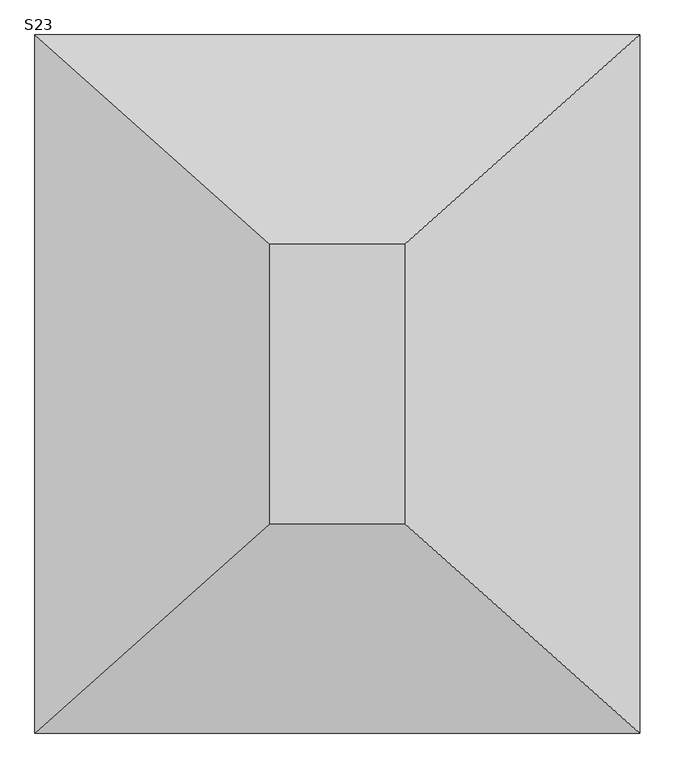
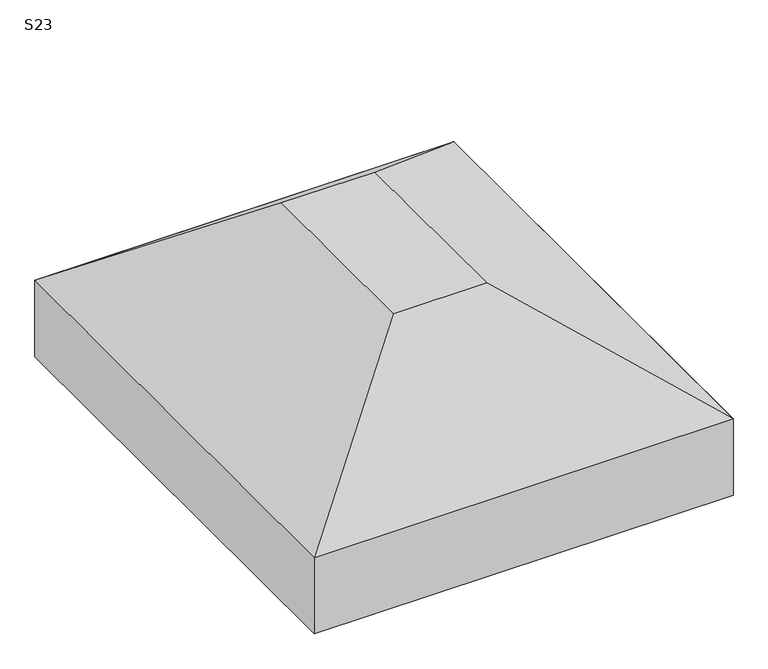
"""IFC4 building model written with IfcOpenShell, lengths in millimetres: fastener geometry, TQS - Sapata : S23."""

import ifcopenshell
import ifcopenshell.guid

model = None  # the IFC model being written
_history = None  # IfcOwnerHistory: only IFC2X3 demands one
_inside = {}  # id of a spatial element -> (the spatial element, [elements in it])
_under = {}  # id of a project, library or spatial element -> (it, [spatial elements below it])
_declared = {}  # id of a project -> (the project, [libraries it declares])
_typed = {}  # id of a type object -> (the type object, [elements of that type])
_made_of = {}  # id of a material, layer set ... -> (it, [elements and type objects made of it])


def new_model(schema):
    """Start an empty IFC model of exactly this schema.

    Asked for "IFC4X3", IfcOpenShell would pick the latest addendum, in which some entities
    have other attributes; the version numbers below select the first issue.
    IFC2X3 requires an IfcOwnerHistory on every rooted entity: one is made here for all.
    """
    global model, _history
    if schema == "IFC4X3":
        model = ifcopenshell.file(schema_version=(4, 3, 0, 0))
    else:
        model = ifcopenshell.file(schema=schema)
    _inside.clear()
    _under.clear()
    _declared.clear()
    _typed.clear()
    _made_of.clear()
    _history = None
    if model.schema == "IFC2X3":
        org = make("IfcOrganization", Name="unknown")
        user = make(
            "IfcPersonAndOrganization",
            ThePerson=make("IfcPerson", FamilyName="unknown"),
            TheOrganization=org,
        )
        app = make(
            "IfcApplication",
            ApplicationDeveloper=org,
            Version="unknown",
            ApplicationFullName="unknown",
            ApplicationIdentifier="unknown",
        )
        _history = make(
            "IfcOwnerHistory",
            OwningUser=user,
            OwningApplication=app,
            ChangeAction="ADDED",
            CreationDate=0,
        )
    return model


def make(cls, **values):
    """One entity of the class cls with the attributes given. An attribute that is None is left unset."""
    return model.create_entity(
        cls, **{name: value for name, value in values.items() if value is not None}
    )


def rooted(cls, **values):
    """An entity with a GlobalId (a new one), such as an element, a storey or a relation."""
    return make(cls, GlobalId=ifcopenshell.guid.new(), OwnerHistory=_history, **values)


def si_unit(unit_type, name, prefix=None):
    """IfcSIUnit, for example si_unit("LENGTHUNIT", "METRE", prefix="MILLI")."""
    return make("IfcSIUnit", UnitType=unit_type, Prefix=prefix, Name=name)


def assignment(units):
    """IfcUnitAssignment: the units of a project."""
    return None if units is None else make("IfcUnitAssignment", Units=units)


def point(xyz):
    """IfcCartesianPoint."""
    return None if xyz is None else make("IfcCartesianPoint", Coordinates=xyz)


def direction(xyz):
    """IfcDirection."""
    return None if xyz is None else make("IfcDirection", DirectionRatios=xyz)


def frame(location, z_axis=None, x_axis=None):
    """IfcAxis2Placement3D, a coordinate frame: its origin and axes. An axis left out is left unset."""
    return make(
        "IfcAxis2Placement3D",
        Location=point(location),
        Axis=direction(z_axis),
        RefDirection=direction(x_axis),
    )


def origin():
    """The frame at (0, 0, 0) with its axes left unset."""
    return frame((0.0, 0.0, 0.0))


def place(relative_to, where):
    """IfcLocalPlacement: puts the frame where relative to a parent placement (None: the world)."""
    return make(
        "IfcLocalPlacement", PlacementRelTo=relative_to, RelativePlacement=where
    )


def context(
    kind, dimensions, precision=None, world=None, true_north=None, identifier=None
):
    """IfcGeometricRepresentationContext, for example the 3D "Model" context."""
    return make(
        "IfcGeometricRepresentationContext",
        ContextIdentifier=identifier,
        ContextType=kind,
        CoordinateSpaceDimension=dimensions,
        Precision=precision,
        WorldCoordinateSystem=world,
        TrueNorth=true_north,
    )


def project(units=None, contexts=None):
    """IfcProject with its units and contexts."""
    return rooted(
        "IfcProject",
        Name="project",
        RepresentationContexts=contexts,
        UnitsInContext=assignment(units),
    )


def spatial(cls, under=None, at=None, **own):
    """A site, building, storey or space (cls), placed at a placement, below another one or the project."""
    s = rooted(cls, ObjectPlacement=at, **own)
    if under is not None:
        _under.setdefault(under.id(), (under, []))[1].append(s)
    return s


def polyline(points):
    """IfcPolyline through the points."""
    return make("IfcPolyline", Points=[point(p) for p in points])


def outline(outer, holes=None, kind="AREA"):
    """IfcArbitraryClosedProfileDef: a profile drawn as a closed curve; with holes, ...WithVoids."""
    if holes is None:
        return make("IfcArbitraryClosedProfileDef", ProfileType=kind, OuterCurve=outer)
    return make(
        "IfcArbitraryProfileDefWithVoids",
        ProfileType=kind,
        OuterCurve=outer,
        InnerCurves=holes,
    )


def extrude(swept, where, along, depth):
    """IfcExtrudedAreaSolid: the profile swept, set in the frame where, extruded along a direction by depth."""
    return make(
        "IfcExtrudedAreaSolid",
        SweptArea=swept,
        Position=where,
        ExtrudedDirection=direction(along),
        Depth=depth,
    )


def faces_of(points, faces, orient=None, outer=None):
    """IfcFace entities. A face is a list of loops; a loop is a list of indices into points, from 0.

    orient and outer hold one flag for each loop. By default every Orientation is true, the
    first loop of a face is its IfcFaceOuterBound and the others are IfcFaceBound.
    """
    made = []
    for i, loops in enumerate(faces):
        bounds = []
        for j, loop in enumerate(loops):
            is_outer = j == 0 if outer is None else outer[i][j]
            bounds.append(
                make(
                    "IfcFaceOuterBound" if is_outer else "IfcFaceBound",
                    Bound=make("IfcPolyLoop", Polygon=[points[k] for k in loop]),
                    Orientation=True if orient is None else orient[i][j],
                )
            )
        made.append(make("IfcFace", Bounds=bounds))
    return made


def faceted_brep(points, faces, orient=None, outer=None, voids=None):
    """IfcFacetedBrep: a solid bounded by flat faces; with voids (closed shells), ...WithVoids."""
    shared = [point(p) for p in points]
    hull = make("IfcClosedShell", CfsFaces=faces_of(shared, faces, orient, outer))
    if voids is None:
        return make("IfcFacetedBrep", Outer=hull)
    return make(
        "IfcFacetedBrepWithVoids",
        Outer=hull,
        Voids=[
            make(cls, CfsFaces=faces_of(shared, fs, o, b)) for cls, fs, o, b in voids
        ],
    )


def shape(context_of_items, identifier, shape_type, items):
    """IfcShapeRepresentation: the items that make up one representation, for example the "Body"."""
    return make(
        "IfcShapeRepresentation",
        ContextOfItems=context_of_items,
        RepresentationIdentifier=identifier,
        RepresentationType=shape_type,
        Items=items,
    )


def source(mapping_origin, context_of_items, identifier, shape_type, items):
    """IfcRepresentationMap: a shape defined once, which mapped items show again and again."""
    return make(
        "IfcRepresentationMap",
        MappingOrigin=mapping_origin,
        MappedRepresentation=shape(context_of_items, identifier, shape_type, items),
    )


def transform(
    local_origin,
    x_axis=None,
    y_axis=None,
    z_axis=None,
    scale=None,
    scale2=None,
    scale3=None,
    uniform=True,
):
    """IfcCartesianTransformationOperator3D, or its non-uniform kind. x_axis, y_axis, z_axis: its Axis1, 2, 3."""
    if uniform:
        return make(
            "IfcCartesianTransformationOperator3D",
            Axis1=direction(x_axis),
            Axis2=direction(y_axis),
            LocalOrigin=point(local_origin),
            Scale=scale,
            Axis3=direction(z_axis),
        )
    return make(
        "IfcCartesianTransformationOperator3DnonUniform",
        Axis1=direction(x_axis),
        Axis2=direction(y_axis),
        LocalOrigin=point(local_origin),
        Scale=scale,
        Axis3=direction(z_axis),
        Scale2=scale2,
        Scale3=scale3,
    )


def mapped(mapping_source, mapping_target):
    """IfcMappedItem: shows the shape of a source again, moved by a transform."""
    return make(
        "IfcMappedItem", MappingSource=mapping_source, MappingTarget=mapping_target
    )


def made_of(thing, what):
    """Note that an element or type object is made of a material, layer set ...; save() writes the relation."""
    if what is not None:
        _made_of.setdefault(what.id(), (what, []))[1].append(thing)
    return thing


def element(
    cls,
    number,
    at=None,
    inside=None,
    cuts=None,
    type_object=None,
    material=None,
    context=None,
    identifier="Body",
    shape_type=None,
    held_by="IfcProductDefinitionShape",
    body=None,
    shapes=None,
    **own,
):
    """One element of the class cls, such as IfcWall. Its Tag is "e" and its number.

    at: its placement. inside: the storey or other place that contains it. cuts: it is an
    opening in that element (IfcRelVoidsElement). A single representation is given by context,
    identifier, shape_type and body (its items); several are given by shapes. held_by: the class
    of the entity that holds the representations. save() writes the other relations.
    """
    e = rooted(cls, Tag="e%d" % number, ObjectPlacement=at, **own)
    if body is not None:
        shapes = [shape(context, identifier, shape_type, body)]
    if shapes is not None:
        e.Representation = make(held_by, Representations=shapes)
    if inside is not None:
        _inside.setdefault(inside.id(), (inside, []))[1].append(e)
    if cuts is not None:
        rooted(
            "IfcRelVoidsElement", RelatingBuildingElement=cuts, RelatedOpeningElement=e
        )
    if type_object is not None:
        _typed.setdefault(type_object.id(), (type_object, []))[1].append(e)
    return made_of(e, material)


def aggregate(whole, parts):
    """IfcRelAggregates: a whole, such as a stair, and the parts it consists of."""
    return rooted("IfcRelAggregates", RelatingObject=whole, RelatedObjects=parts)


def save(model, path):
    """Write the relations noted so far, then the file.

    IfcRelAggregates (storeys below a building ...), IfcRelContainedInSpatialStructure (elements
    in a storey), IfcRelDefinesByType, IfcRelAssociatesMaterial and IfcRelDeclares: one each for
    every whole, place, type object, material and project.
    """
    for whole, parts in _under.values():
        aggregate(whole, parts)
    for where, things in _inside.values():
        rooted(
            "IfcRelContainedInSpatialStructure",
            RelatedElements=things,
            RelatingStructure=where,
        )
    for kind, things in _typed.values():
        rooted("IfcRelDefinesByType", RelatedObjects=things, RelatingType=kind)
    for what, things in _made_of.values():
        rooted("IfcRelAssociatesMaterial", RelatedObjects=things, RelatingMaterial=what)
    for by, libraries in _declared.values():
        rooted("IfcRelDeclares", RelatingContext=by, RelatedDefinitions=libraries)
    model.write(path)


def s23_c1a85685(model_context):
    return source(origin(), model_context, "Body", "SolidModel", [
        faceted_brep([(-55.0, 100.0, 0.0), (-345.0, 100.0, 0.0), (-345.0, -500.0, 0.0), (-55.0, -500.0, 0.0), (450.0, 550.0, -350.0), (450.0, -950.0, -350.0), (-850.0, -950.0, -350.0), (-850.0, 550.0, -350.0)], [[[0, 1, 2, 3]], [[4, 5, 6, 7]], [[4, 7, 1, 0]], [[7, 6, 2, 1]], [[6, 5, 3, 2]], [[5, 4, 0, 3]]]),
        extrude(outline(polyline([(450.0, 550.0), (450.0, -950.0), (-850.0, -950.0), (-850.0, 550.0), (450.0, 550.0)])), frame((0.0, 0.0, -600.0), z_axis=(0.0, 0.0, 1.0), x_axis=(1.0, 0.0, 0.0)), (0.0, 0.0, 1.0), 250.0),
    ])


if __name__ == "__main__":
    model = new_model("IFC4")
    model_context = context("Model", 3, world=origin())
    ifc_project = project(units=[si_unit("LENGTHUNIT", "METRE", prefix="MILLI")], contexts=[model_context])
    site = spatial("IfcSite", under=ifc_project)
    building = spatial("IfcBuilding", under=site)
    placement = place(None, origin())
    s23_shape = s23_c1a85685(model_context)
    element("IfcFastener", 1, ObjectType="TQS - Sapata : S23", at=placement, inside=building, context=model_context, shape_type="MappedRepresentation", body=[
        mapped(s23_shape, transform((0.0, 0.0, 0.0), x_axis=(1.0, 0.0, 0.0), y_axis=(0.0, 1.0, 0.0), z_axis=(0.0, 0.0, 1.0))),
    ])
    save(model, "model.ifc")

# Revit data of these elements
# Type "TQS - Sapata : S23"
#   TY = 0.60 m
#   TX = 0.29 m
#   HS = 0.60 m
#   H0 = 0.25 m
#   EXCYABS = 0.75 m
#   EXCY = 0.00 m
#   EXCXABS = 0.65 m
#   EXCX = 0.00 m
#   DIMY = 1.50 m
#   DIMX = 1.30 m
#   Material estrutural = Concreto - Concreto concretado no local
#   Width = 0
#   Length = 0
# Element 1 (IfcFastener, "TQS - Sapata : S23")
#   Materials on its faces: "Concreto - Concreto concretado no local"
# Materials
#   "Concreto - Concreto concretado no local": class "Concreto", colour RGB 192 192 192, transparency 0
